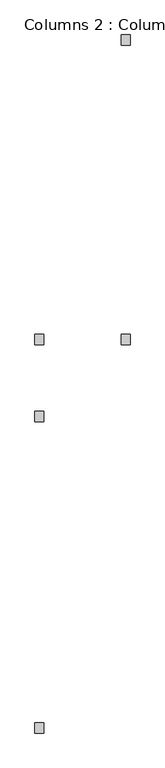
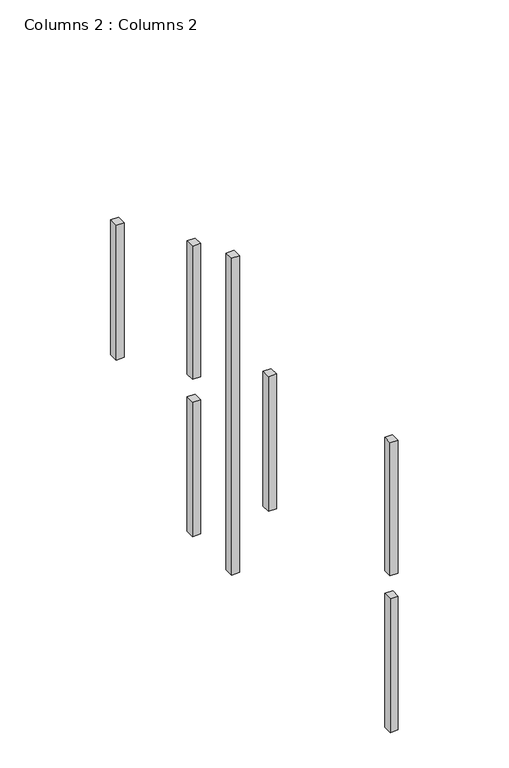
"""IFC4 building model written with IfcOpenShell, lengths in millimetres: column geometry, Columns 2 : Columns 2."""

from ifc_helpers import new_model, si_unit, frame, origin, place, context, project, spatial, polyline, outline, extrude, source, transform, mapped, element, save


def columns_2_columns_2_bbcb63ce(model_context):
    return source(origin(), model_context, "Body", "SweptSolid", [
        extrude(outline(polyline([(31910.3221032, 36331.2207942), (31910.3221032, 36483.6207942), (32040.4971032, 36483.6207942), (32040.4971032, 36331.2207942), (31910.3221032, 36331.2207942)])), frame((0.0, 0.0, 269146.3375), z_axis=(0.0, 0.0, 1.0), x_axis=(1.0, 0.0, 0.0)), (0.0, 0.0, 1.0), 2316.1625),
        extrude(outline(polyline([(31910.3221032, 35213.6207942), (31910.3221032, 35366.0207942), (32040.4971032, 35366.0207942), (32040.4971032, 35213.6207942), (31910.3221032, 35213.6207942)])), frame((0.0, 0.0, 266422.1875), z_axis=(0.0, 0.0, 1.0), x_axis=(1.0, 0.0, 0.0)), (0.0, 0.0, 1.0), 5505.45),
        extrude(outline(polyline([(33159.6965778, 40668.9106612), (33159.6965778, 40821.3106612), (33289.8715778, 40821.3106612), (33289.8715778, 40668.9106612), (33159.6965778, 40668.9106612)])), frame((0.0, 0.0, 266414.25), z_axis=(0.0, 0.0, 1.0), x_axis=(1.0, 0.0, 0.0)), (0.0, 0.0, 1.0), 2343.15),
        extrude(outline(polyline([(33159.6965778, 36331.2207942), (33159.6965778, 36483.6207942), (33289.8715778, 36483.6207942), (33289.8715778, 36331.2207942), (33159.6965778, 36331.2207942)])), frame((0.0, 0.0, 266414.25), z_axis=(0.0, 0.0, 1.0), x_axis=(1.0, 0.0, 0.0)), (0.0, 0.0, 1.0), 2343.15),
        extrude(outline(polyline([(31911.9215778, 36331.2207942), (31911.9215778, 36483.6207942), (32042.0965778, 36483.6207942), (32042.0965778, 36331.2207942), (31911.9215778, 36331.2207942)])), frame((0.0, 0.0, 266414.25), z_axis=(0.0, 0.0, 1.0), x_axis=(1.0, 0.0, 0.0)), (0.0, 0.0, 1.0), 2335.2125),
        extrude(outline(polyline([(31910.3221032, 30698.1406612), (31910.3221032, 30850.5406612), (32040.4971032, 30850.5406612), (32040.4971032, 30698.1406612), (31910.3221032, 30698.1406612)])), frame((0.0, 0.0, 269146.3375), z_axis=(0.0, 0.0, 1.0), x_axis=(1.0, 0.0, 0.0)), (0.0, 0.0, 1.0), 2316.1625),
        extrude(outline(polyline([(31911.9215778, 30698.1406612), (31911.9215778, 30850.5406612), (32042.0965778, 30850.5406612), (32042.0965778, 30698.1406612), (31911.9215778, 30698.1406612)])), frame((0.0, 0.0, 266422.1875), z_axis=(0.0, 0.0, 1.0), x_axis=(1.0, 0.0, 0.0)), (0.0, 0.0, 1.0), 2327.275),
    ])


if __name__ == "__main__":
    model = new_model("IFC4")
    model_context = context("Model", 3, world=origin())
    ifc_project = project(units=[si_unit("LENGTHUNIT", "METRE", prefix="MILLI")], contexts=[model_context])
    site = spatial("IfcSite", under=ifc_project)
    building = spatial("IfcBuilding", under=site)
    placement = place(None, origin())
    columns_2_columns_2_shape = columns_2_columns_2_bbcb63ce(model_context)
    element("IfcColumn", 1, ObjectType="Columns 2 : Columns 2", at=placement, inside=building, context=model_context, shape_type="MappedRepresentation", body=[
        mapped(columns_2_columns_2_shape, transform((0.0, 0.0, 0.0), x_axis=(1.0, 0.0, 0.0), y_axis=(0.0, 1.0, 0.0), z_axis=(0.0, 0.0, 1.0))),
    ])
    save(model, "model.ifc")

# Revit data of these elements
# Element 1 (IfcColumn, "Columns 2 : Columns 2")
#   Materials on its faces: "5 1/8\" x 6\" GLUELAM COLUMN"
# Materials
#   "5 1/8\" x 6\" GLUELAM COLUMN": class "Wood", colour RGB 144 113 62, transparency 0, Description = "Pinus Echinata", Cost = 0
